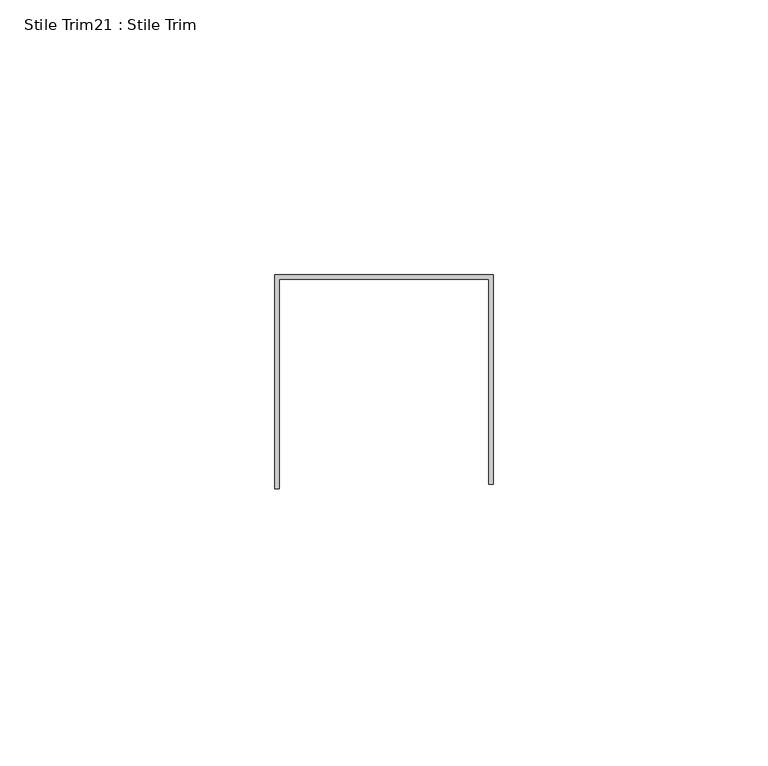
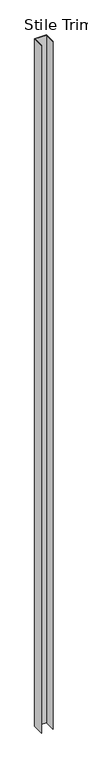
"""IFC4 building model written with IfcOpenShell, lengths in millimetres: proxy geometry, Stile Trim21 : Stile Trim."""

from ifc_helpers import new_model, si_unit, frame, origin, place, context, project, spatial, polyline, outline, extrude, source, transform, mapped, element, save


def stile_trim21_stile_trim_282884a6(model_context):
    return source(origin(), model_context, "Body", "SweptSolid", [
        extrude(outline(polyline([(587327.0060739, -536293.7663841), (587366.6808739, -536293.7663841), (587366.6808739, -536331.8663841), (587365.8934739, -536331.8663841), (587365.8934739, -536294.5537841), (587327.7934739, -536294.5537841), (587327.7934739, -536332.6537841), (587327.0060739, -536332.6537841), (587327.0060739, -536293.7663841)])), frame((0.0, 0.0, 12.7), z_axis=(0.0, 0.0, 1.0), x_axis=(1.0, 0.0, 0.0)), (0.0, 0.0, 1.0), 2425.7),
    ])


if __name__ == "__main__":
    model = new_model("IFC4")
    model_context = context("Model", 3, world=origin())
    ifc_project = project(units=[si_unit("LENGTHUNIT", "METRE", prefix="MILLI")], contexts=[model_context])
    site = spatial("IfcSite", under=ifc_project)
    building = spatial("IfcBuilding", under=site)
    placement = place(None, origin())
    stile_trim21_stile_trim_shape = stile_trim21_stile_trim_282884a6(model_context)
    element("IfcBuildingElementProxy", 1, Name="Stile Trim21 : Stile Trim", ObjectType="Stile Trim21 : Stile Trim", at=placement, inside=building, context=model_context, shape_type="MappedRepresentation", body=[
        mapped(stile_trim21_stile_trim_shape, transform((0.0, 0.0, 0.0), x_axis=(1.0, 0.0, 0.0), y_axis=(0.0, 1.0, 0.0), z_axis=(0.0, 0.0, 1.0))),
    ])
    save(model, "model.ifc")

# Revit data of these elements
# Element 1 (IfcBuildingElementProxy, "Stile Trim21 : Stile Trim")
#   Materials on its faces: "EDGE TRIM BY MTL PANEL MFR."
# Materials
#   "EDGE TRIM BY MTL PANEL MFR.": class "Generic", colour RGB 239 242 240, transparency 0, Cost = 0
